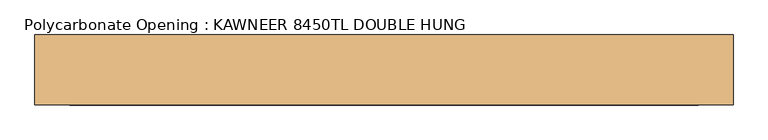
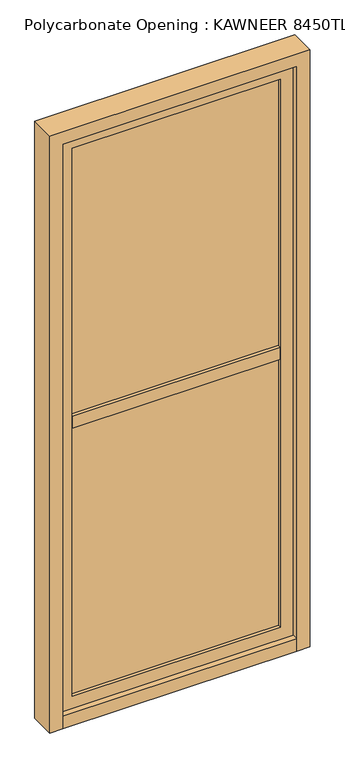
"""IFC4 building model written with IfcOpenShell, lengths in millimetres: door geometry, Polycarbonate Opening : KAWNEER 8450TL DOUBLE HUNG."""

from ifc_helpers import new_model, si_unit, frame, origin, origin_with_axes, place, context, project, spatial, polyline, outline, extrude, source, transform, mapped, element, save


def polycarbonate_opening_kawneer_8450tl_double_hung_e4587749(model_context):
    return source(origin(), model_context, "Body", "SweptSolid", [
        extrude(outline(polyline([(457.2, 12.7), (457.2, -12.7), (-457.2, -12.7), (-457.2, 12.7), (457.2, 12.7)])), frame((0.0, 0.0, 50.8), z_axis=(0.0, 0.0, 1.0), x_axis=(1.0, 0.0, 0.0)), (0.0, 0.0, 1.0), 2360.0132885),
        extrude(outline(polyline([(2410.8132885, -457.2), (0.0, -457.2), (0.0, 457.2), (2410.8132885, 457.2), (2410.8132885, -457.2)]), holes=[polyline([(101.6, 406.4), (101.6, -406.4), (2360.0132885, -406.4), (2360.0132885, 406.4), (101.6, 406.4)])]), frame((0.0, -25.4, 0.0), z_axis=(0.0, 1.0, 0.0), x_axis=(0.0, 0.0, 1.0)), (0.0, 0.0, 1.0), 50.8),
        extrude(outline(polyline([(2461.6132885, 508.0), (2461.6132885, -508.0), (0.0, -508.0), (0.0, -457.2), (2410.8132885, -457.2), (2410.8132885, 457.2), (0.0, 457.2), (0.0, 508.0), (2461.6132885, 508.0)])), frame((0.0, -50.8, 0.0), z_axis=(0.0, 1.0, 0.0), x_axis=(0.0, 0.0, 1.0)), (0.0, 0.0, 1.0), 101.6),
        extrude(outline(polyline([(457.2, 50.8), (457.2, -50.8), (-457.2, -50.8), (-457.2, 50.8), (457.2, 50.8)])), origin_with_axes(), (0.0, 0.0, 1.0), 50.8),
        extrude(outline(polyline([(406.4, 25.4), (406.4, -25.4), (-406.4, -25.4), (-406.4, 25.4), (406.4, 25.4)])), frame((0.0, 0.0, 1205.4066443), z_axis=(0.0, 0.0, 1.0), x_axis=(1.0, 0.0, 0.0)), (0.0, 0.0, 1.0), 50.8),
    ])


if __name__ == "__main__":
    model = new_model("IFC4")
    model_context = context("Model", 3, world=origin())
    ifc_project = project(units=[si_unit("LENGTHUNIT", "METRE", prefix="MILLI")], contexts=[model_context])
    site = spatial("IfcSite", under=ifc_project)
    building = spatial("IfcBuilding", under=site)
    placement = place(None, origin())
    polycarbonate_opening_kawneer_8450tl_double_hung_shape = polycarbonate_opening_kawneer_8450tl_double_hung_e4587749(model_context)
    element("IfcDoor", 1, ObjectType="Polycarbonate Opening : KAWNEER 8450TL DOUBLE HUNG", at=placement, inside=building, context=model_context, shape_type="MappedRepresentation", body=[
        mapped(polycarbonate_opening_kawneer_8450tl_double_hung_shape, transform((0.0, 0.0, 0.0), x_axis=(1.0, 0.0, 0.0), y_axis=(0.0, 1.0, 0.0), z_axis=(0.0, 0.0, 1.0))),
    ])
    save(model, "model.ifc")

# Revit data of these elements
# Type "Polycarbonate Opening : KAWNEER 8450TL DOUBLE HUNG"
#   Type Mark = "59"
#   OD_DS_Door_Material = "ALUM./GLAZING"
#   OD_DS_Door_Type = "STOREFRONT - DOUBLE HUNG WINDOW"
#   OD_DS_Lockset = "POLE OPERATOR HARDWARE FOR TOP SASH; BOTTOM SASH MECHANICALLY FIXED"
#   Analytic Construction = "<None>"
#   offset [instance default] = 0' - 2"
#   Stile = 0' - 2"
#   Mullion Width = 0' - 2"
#   Mullion Depth = 0' - 4"
#   Opening Size [instance default] = 5' - 1.50212"
#   Door Width [instance default] = 5' - 1.50212"
#   Window ON/OFF = no
#   Door On/Off = yes
#   Mullion Material = DOUBLE HUNG (CLEAR ANODIZED ALUM) - TEMPERED INSULATED GLAZING (CARDINAL GLASS LoĒ²-240\nOR EQUIVALENT)
#   Glass Material = TEMPERED INSULATED GLAZING (CARDINAL GLASS LoĒ²-240\nOR EQUIVALENT)
#   Door Material = DOUBLE HUNG (CLEAR ANODIZED ALUM) - TEMPERED INSULATED GLAZING (CARDINAL GLASS LoĒ²-240\nOR EQUIVALENT)
# Element 1 (IfcDoor, "Polycarbonate Opening : KAWNEER 8450TL DOUBLE HUNG")
#   offset = 0' - 0"
#   Materials on its faces: "DOUBLE HUNG (CLEAR ANODIZED ALUM) - TEMPERED INSULATED GLAZING (CARDINAL GLASS LoĒ²-240\nOR EQUIVALENT)", "TEMPERED INSULATED GLAZING (CARDINAL GLASS LoĒ²-240\nOR EQUIVALENT)"
# Materials
#   "DOUBLE HUNG (CLEAR ANODIZED ALUM) - TEMPERED INSULATED GLAZING (CARDINAL GLASS LoĒ²-240\nOR EQUIVALENT)": class "Metal", colour RGB 244 244 244, transparency 0, Description = "Aluminum 6061", Cost = 0
#   "TEMPERED INSULATED GLAZING (CARDINAL GLASS LoĒ²-240\nOR EQUIVALENT)": class "Glass", colour RGB 196 205 210, transparency 0.85, Description = "Soda Lime Glass", Cost = 0
